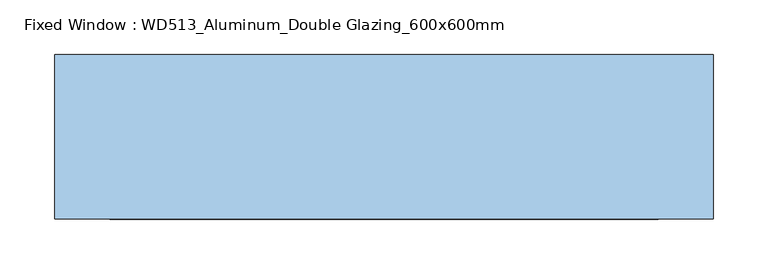
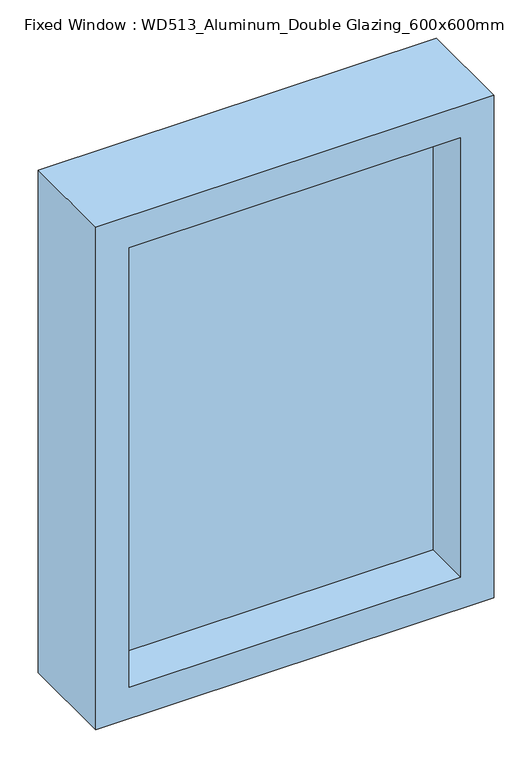
"""IFC4 building model written with IfcOpenShell, lengths in millimetres: window geometry, Fixed Window : WD513_Aluminum_Double Glazing_600x600mm."""

from ifc_helpers import new_model, si_unit, frame, origin, place, context, project, spatial, polyline, outline, extrude, source, transform, mapped, element, save


def fixed_window_wd513_aluminum_double_glazing_600x600mm_37dd25d6(model_context):
    return source(origin(), model_context, "Body", "SweptSolid", [
        extrude(outline(polyline([(-250.0, 3.0), (250.0, 3.0), (250.0, -3.0), (-250.0, -3.0), (-250.0, 3.0)])), frame((0.0, 0.0, 850.0), z_axis=(0.0, 0.0, 1.0), x_axis=(1.0, 0.0, 0.0)), (0.0, 0.0, 1.0), 700.0),
        extrude(outline(polyline([(1600.0, -300.0), (800.0, -300.0), (800.0, 300.0), (1600.0, 300.0), (1600.0, -300.0)]), holes=[polyline([(1550.0, -250.0), (1550.0, 250.0), (850.0, 250.0), (850.0, -250.0), (1550.0, -250.0)])]), frame((0.0, -75.0, 0.0), z_axis=(0.0, 1.0, 0.0), x_axis=(0.0, 0.0, 1.0)), (0.0, 0.0, 1.0), 150.0),
    ])


if __name__ == "__main__":
    model = new_model("IFC4")
    model_context = context("Model", 3, world=origin())
    ifc_project = project(units=[si_unit("LENGTHUNIT", "METRE", prefix="MILLI")], contexts=[model_context])
    site = spatial("IfcSite", under=ifc_project)
    building = spatial("IfcBuilding", under=site)
    placement = place(None, origin())
    fixed_window_wd513_aluminum_double_glazing_600x600mm_shape = fixed_window_wd513_aluminum_double_glazing_600x600mm_37dd25d6(model_context)
    element("IfcWindow", 1, ObjectType="Fixed Window : WD513_Aluminum_Double Glazing_600x600mm", at=placement, inside=building, context=model_context, shape_type="MappedRepresentation", body=[
        mapped(fixed_window_wd513_aluminum_double_glazing_600x600mm_shape, transform((0.0, 0.0, 0.0), x_axis=(1.0, 0.0, 0.0), y_axis=(0.0, 1.0, 0.0), z_axis=(0.0, 0.0, 1.0))),
    ])
    save(model, "model.ifc")

# Revit data of these elements
# Type "Fixed Window : WD513_Aluminum_Double Glazing_600x600mm"
#   Type Mark = "AW"
#   Analytic Construction = "<None>"
#   창 두께 = 150 mm
#   Height = 800 mm
#   절반 창 두께 = 75 mm
#   기본 씰 높이 = 800 mm
#   Width = 600 mm
#   Define Thermal Properties by = 1
#   창 패널 = AW2 창 패널
#   창 프레임 = A04AQ127-00002_Aluminum Window_None FP
#   Wall Closure = (empty or 0)
# Element 1 (IfcWindow, "Fixed Window : WD513_Aluminum_Double Glazing_600x600mm")
#   Materials on its faces: "A04AQ127-00002_Aluminum Window_None FP", "AW2 창 패널"
# Materials
#   "AW2 창 패널": class "유리", colour RGB 0 0 255, transparency 0.75
#   "A04AQ127-00002_Aluminum Window_None FP": class "금속", colour RGB 247 247 247, transparency 0, W00) Work Master Code = "A04AQ127-00002", W01) Work Master_Lv1 = "Finishing Work", W02) Work Master_Lv2 = "Door & Window Work", W03) Work Master_Spec.1 = "Aluminum Window", W04) Work Master_Spec.2 = "Fire Protective Rating: N/A", W05) Work Master_Spec.3 = "w/ Hardware & Accessories", Cost = 0
